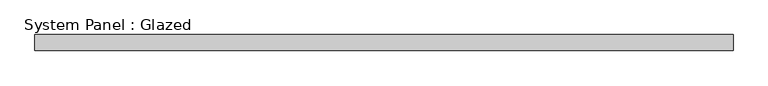
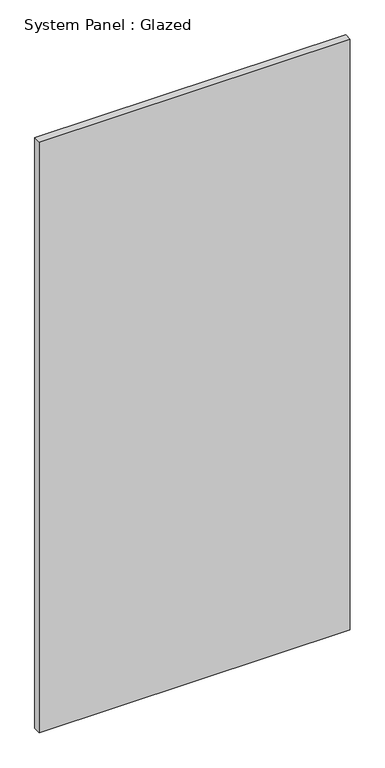
"""IFC4 building model written with IfcOpenShell, lengths in millimetres: plate geometry, System Panel : Glazed."""

from ifc_helpers import new_model, si_unit, origin, origin_with_axes, place, context, project, spatial, polyline, outline, extrude, source, transform, mapped, element, save


def system_panel_glazed_578ed88e(model_context):
    return source(origin(), model_context, "Body", "SweptSolid", [
        extrude(outline(polyline([(551.965768, -44.45), (-551.965768, -44.45), (-551.965768, -19.05), (551.965768, -19.05), (551.965768, -44.45)])), origin_with_axes(), (0.0, 0.0, 1.0), 2216.15),
    ])


if __name__ == "__main__":
    model = new_model("IFC4")
    model_context = context("Model", 3, world=origin())
    ifc_project = project(units=[si_unit("LENGTHUNIT", "METRE", prefix="MILLI")], contexts=[model_context])
    site = spatial("IfcSite", under=ifc_project)
    building = spatial("IfcBuilding", under=site)
    placement = place(None, origin())
    system_panel_glazed_shape = system_panel_glazed_578ed88e(model_context)
    element("IfcPlate", 1, ObjectType="System Panel : Glazed", at=placement, inside=building, context=model_context, shape_type="MappedRepresentation", body=[
        mapped(system_panel_glazed_shape, transform((0.0, 0.0, 0.0), x_axis=(1.0, 0.0, 0.0), y_axis=(0.0, 1.0, 0.0), z_axis=(0.0, 0.0, 1.0))),
    ])
    save(model, "model.ifc")

# Revit data of these elements
# Type "System Panel : Glazed"
#   Construction Type Id = "GSP4R"
#   Analytic Construction = "1/8 in Pilkington single glazing"
#   Visual Light Transmittance = 0.9
#   Solar Heat Gain Coefficient = 0.86
#   Heat Transfer Coefficient (U) = 1.18115 BTU/(h·ft²·°F)
#   Define Thermal Properties by = 1
# Element 1 (IfcPlate, "System Panel : Glazed")
#   Materials on its faces: "Glass"
# Materials
#   "Glass": class "Glass", colour RGB 0 128 192, transparency 0.75, Description = "Soda Lime Glass", Cost = 0
